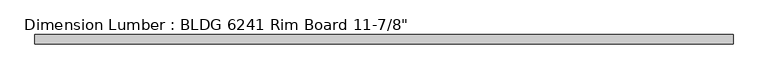
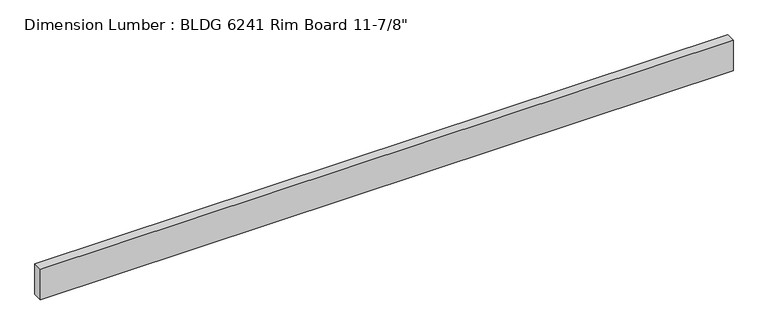
"""IFC4 building model written with IfcOpenShell, lengths in millimetres: beam geometry."""

from ifc_helpers import new_model, si_unit, frame, origin, place, context, project, spatial, polyline, outline, extrude, source, transform, mapped, element, save


def beam_440427b1(model_context):
    return source(origin(), model_context, "Body", "SweptSolid", [
        extrude(outline(polyline([(3254.375, 44.45), (3254.375, -44.45), (-3254.375, -44.45), (-3254.375, 44.45), (3254.375, 44.45)])), frame((0.0, 0.0, -150.8125), z_axis=(0.0, 0.0, 1.0), x_axis=(1.0, 0.0, 0.0)), (0.0, 0.0, 1.0), 301.625),
    ])


if __name__ == "__main__":
    model = new_model("IFC4")
    model_context = context("Model", 3, world=origin())
    ifc_project = project(units=[si_unit("LENGTHUNIT", "METRE", prefix="MILLI")], contexts=[model_context])
    site = spatial("IfcSite", under=ifc_project)
    building = spatial("IfcBuilding", under=site)
    placement = place(None, origin())
    beam_shape = beam_440427b1(model_context)
    element("IfcBeam", 1, ObjectType="Dimension Lumber : BLDG 6241 Rim Board 11-7/8\"", at=placement, inside=building, context=model_context, shape_type="MappedRepresentation", body=[
        mapped(beam_shape, transform((0.0, 0.0, 0.0), x_axis=(1.0, 0.0, 0.0), y_axis=(0.0, 1.0, 0.0), z_axis=(0.0, 0.0, 1.0))),
    ])
    save(model, "model.ifc")

# Revit data of these elements
# Type "Dimension Lumber : BLDG 6241 Rim Board 11-7/8\""
#   Assembly Code = "B10"
#   A = 0.273472 SF
#   Length [instance default] = 5' - 0"
#   b = 0' - 3 1/2"
#   d = 0' - 11 7/8"
#   Structural Material [instance default] = Softwood, Lumber
# Element 1 (IfcBeam, "Dimension Lumber : BLDG 6241 Rim Board 11-7/8\"")
#   Materials on its faces: "Softwood, Lumber"
# Materials
#   "Softwood, Lumber": class "Wood", colour RGB 223 192 134, transparency 0, Description = "Pinus Echinata", Cost = 0
